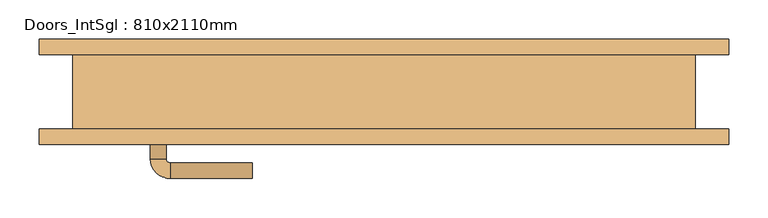
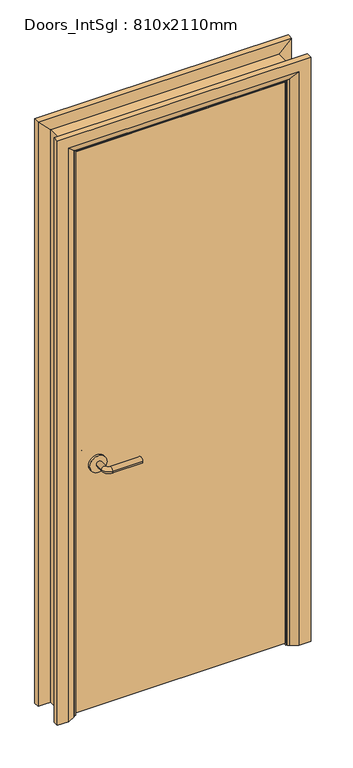
"""IFC4 building model written with IfcOpenShell, lengths in millimetres: door geometry, Doors_IntSgl : 810x2110mm."""

from ifc_helpers import new_model, si_unit, point, frame, frame_2d, origin, place, context, project, spatial, polyline, circle_curve, ellipse_curve, trimmed, segment, composite_curve, outline, extrude, faceted_brep, source, transform, mapped, element, save
from ifc_brep_helpers import plane_surface, cylinder_surface, revolved_surface, advanced_brep


def doors_intsgl_810x2110mm_4fdc4f61(model_context):
    return source(origin(), model_context, "Body", "SolidModel", [
        advanced_brep(
        [(-298.0, -1.5, 900.0), (-278.0, -1.5, 900.0), (-298.0, 28.5, 900.0), (-278.0, 28.5, 900.0), (-273.0, 33.5, 900.0), (-273.0, 53.5, 900.0), (-168.0, 53.5, 900.0), (-168.0, 33.5, 900.0)],
        [
            (0, 1, circle_curve(frame((-288.0, -1.5, 900.0), z_axis=(0.0, -1.0, 0.0), x_axis=(1.0, 0.0, 0.0)), 10.0)),
            (1, 0, circle_curve(frame((-288.0, -1.5, 900.0), z_axis=(0.0, -1.0, 0.0), x_axis=(1.0, 0.0, 0.0)), 10.0)),
            (0, 2),
            (2, 3, circle_curve(frame((-288.0, 28.5, 900.0), z_axis=(0.0, -1.0, 0.0), x_axis=(1.0, 0.0, 0.0)), 10.0)),
            (3, 1),
            (3, 2, circle_curve(frame((-288.0, 28.5, 900.0), z_axis=(0.0, -1.0, 0.0), x_axis=(1.0, 0.0, 0.0)), 10.0)),
            (4, 3, circle_curve(frame((-273.0, 28.5, 900.0), z_axis=(0.0, 0.0, 1.0), x_axis=(-1.0, 0.0, 0.0)), 5.0)),
            (2, 5, circle_curve(frame((-273.0, 28.5, 900.0), z_axis=(0.0, 0.0, -1.0), x_axis=(-1.0, 0.0, 0.0)), 25.0)),
            (5, 4, circle_curve(frame((-273.0, 43.5, 900.0), z_axis=(-1.0, 0.0, 0.0), x_axis=(0.0, -1.0, 0.0)), 10.0)),
            (4, 5, circle_curve(frame((-273.0, 43.5, 900.0), z_axis=(-1.0, 0.0, 0.0), x_axis=(0.0, -1.0, 0.0)), 10.0)),
            (6, 7, circle_curve(frame((-168.0, 43.5, 900.0), z_axis=(1.0, 0.0, 0.0), x_axis=(0.0, -1.0, 0.0)), 10.0)),
            (7, 6, circle_curve(frame((-168.0, 43.5, 900.0), z_axis=(1.0, 0.0, 0.0), x_axis=(0.0, -1.0, 0.0)), 10.0)),
            (5, 6),
            (7, 4),
        ],
        [
            plane_surface(frame((-288.0, -1.5, 900.0), z_axis=(0.0, -1.0, 0.0), x_axis=(0.0, 0.0, 1.0))),
            cylinder_surface(frame((-288.0, -1.5, 900.0), z_axis=(0.0, -1.0, 0.0), x_axis=(1.0, 0.0, 0.0)), 10.0),
            revolved_surface(trimmed(ellipse_curve(frame((-288.0, 28.5, 900.0), z_axis=(0.0, -1.0, 0.0), x_axis=(1.0, 0.0, 0.0)), 10.0, 10.0), [point((-298.0, 28.5, 900.0))], [point((-278.0, 28.5, 900.0))], True, "CARTESIAN"), (-273.0, 28.5, 900.0), (0.0, 0.0, -1.0)),
            revolved_surface(trimmed(ellipse_curve(frame((-288.0, 28.5, 900.0), z_axis=(0.0, -1.0, 0.0), x_axis=(1.0, 0.0, 0.0)), 10.0, 10.0), [point((-278.0, 28.5, 900.0))], [point((-298.0, 28.5, 900.0))], True, "CARTESIAN"), (-273.0, 28.5, 900.0), (0.0, 0.0, -1.0)),
            plane_surface(frame((-168.0, 43.5, 900.0), z_axis=(1.0, 0.0, 0.0), x_axis=(0.0, 0.0, 1.0))),
            cylinder_surface(frame((-273.0, 43.5, 900.0), z_axis=(-1.0, 0.0, 0.0), x_axis=(0.0, -1.0, 0.0)), 10.0),
        ],
        [
            (0, [[1, 2]]),
            (1, [[-1, 3, 4, 5]]),
            (1, [[-2, -5, 6, -3]]),
            (2, [[7, -4, 8, 9]]),
            (3, [[-8, -6, -7, 10]]),
            (4, [[11, 12]]),
            (5, [[-9, 13, -12, 14]]),
            (5, [[-10, -14, -11, -13]]),
        ],
    ),
        extrude(outline(composite_curve([segment(trimmed(circle_curve(frame_2d((900.0, -290.5)), 30.0), [point((900.0, -320.5))], [point((900.0, -260.5))], False, "CARTESIAN"), True, "CONTINUOUS"), segment(trimmed(circle_curve(frame_2d((900.0, -290.5)), 30.0), [point((900.0, -260.5))], [point((900.0, -320.5))], False, "CARTESIAN"), True, "CONTINUOUS")], self_intersect=False)), frame((0.0, -9.5, 0.0), z_axis=(0.0, 1.0, 0.0), x_axis=(0.0, 0.0, 1.0)), (0.0, 0.0, 1.0), 8.0),
        advanced_brep(
        [(-298.0, -55.5, 900.0), (-278.0, -55.5, 900.0), (-278.0, -85.5, 900.0), (-298.0, -85.5, 900.0), (-273.0, -90.5, 900.0), (-273.0, -110.5, 900.0), (-168.0, -110.5, 900.0), (-168.0, -90.5, 900.0)],
        [
            (0, 1, circle_curve(frame((-288.0, -55.5, 900.0), z_axis=(0.0, 1.0, 0.0), x_axis=(1.0, 0.0, 0.0)), 10.0)),
            (1, 0, circle_curve(frame((-288.0, -55.5, 900.0), z_axis=(0.0, 1.0, 0.0), x_axis=(1.0, 0.0, 0.0)), 10.0)),
            (1, 2),
            (2, 3, circle_curve(frame((-288.0, -85.5, 900.0), z_axis=(0.0, 1.0, 0.0), x_axis=(1.0, 0.0, 0.0)), 10.0)),
            (3, 0),
            (3, 2, circle_curve(frame((-288.0, -85.5, 900.0), z_axis=(0.0, 1.0, 0.0), x_axis=(1.0, 0.0, 0.0)), 10.0)),
            (4, 5, circle_curve(frame((-273.0, -100.5, 900.0), z_axis=(-1.0, 0.0, 0.0), x_axis=(0.0, 1.0, 0.0)), 10.0)),
            (5, 3, circle_curve(frame((-273.0, -85.5, 900.0), z_axis=(0.0, 0.0, -1.0), x_axis=(-1.0, 0.0, 0.0)), 25.0)),
            (2, 4, circle_curve(frame((-273.0, -85.5, 900.0), z_axis=(0.0, 0.0, 1.0), x_axis=(-1.0, 0.0, 0.0)), 5.0)),
            (5, 4, circle_curve(frame((-273.0, -100.5, 900.0), z_axis=(-1.0, 0.0, 0.0), x_axis=(0.0, 1.0, 0.0)), 10.0)),
            (6, 7, circle_curve(frame((-168.0, -100.5, 900.0), z_axis=(1.0, 0.0, 0.0), x_axis=(0.0, 1.0, 0.0)), 10.0)),
            (7, 6, circle_curve(frame((-168.0, -100.5, 900.0), z_axis=(1.0, 0.0, 0.0), x_axis=(0.0, 1.0, 0.0)), 10.0)),
            (4, 7),
            (6, 5),
        ],
        [
            plane_surface(frame((-288.0, -55.5, 900.0), z_axis=(0.0, 1.0, 0.0), x_axis=(0.0, 0.0, 1.0))),
            cylinder_surface(frame((-288.0, -55.5, 900.0), z_axis=(0.0, 1.0, 0.0), x_axis=(1.0, 0.0, 0.0)), 10.0),
            revolved_surface(trimmed(ellipse_curve(frame((-288.0, -85.5, 900.0), z_axis=(0.0, -1.0, 0.0), x_axis=(1.0, 0.0, 0.0)), 10.0, 10.0), [point((-298.0, -85.5, 900.0))], [point((-278.0, -85.5, 900.0))], True, "CARTESIAN"), (-273.0, -85.5, 900.0), (0.0, 0.0, -1.0)),
            revolved_surface(trimmed(ellipse_curve(frame((-288.0, -85.5, 900.0), z_axis=(0.0, -1.0, 0.0), x_axis=(1.0, 0.0, 0.0)), 10.0, 10.0), [point((-278.0, -85.5, 900.0))], [point((-298.0, -85.5, 900.0))], True, "CARTESIAN"), (-273.0, -85.5, 900.0), (0.0, 0.0, -1.0)),
            plane_surface(frame((-168.0, -100.5, 900.0), z_axis=(1.0, 0.0, 0.0), x_axis=(0.0, 0.0, 1.0))),
            cylinder_surface(frame((-273.0, -100.5, 900.0), z_axis=(-1.0, 0.0, 0.0), x_axis=(0.0, 1.0, 0.0)), 10.0),
        ],
        [
            (0, [[1, 2]]),
            (1, [[3, 4, 5, -2]]),
            (1, [[-5, 6, -3, -1]]),
            (2, [[7, 8, -4, 9]]),
            (3, [[10, -9, -6, -8]]),
            (4, [[11, 12]]),
            (5, [[13, -11, 14, -7]]),
            (5, [[-14, -12, -13, -10]]),
        ],
    ),
        extrude(outline(composite_curve([segment(trimmed(circle_curve(frame_2d((900.0, -290.5)), 30.0), [point((900.0, -320.5))], [point((900.0, -260.5))], False, "CARTESIAN"), True, "CONTINUOUS"), segment(trimmed(circle_curve(frame_2d((900.0, -290.5)), 30.0), [point((900.0, -260.5))], [point((900.0, -320.5))], False, "CARTESIAN"), True, "CONTINUOUS")], self_intersect=False)), frame((0.0, -55.5, 0.0), z_axis=(0.0, 1.0, 0.0), x_axis=(0.0, 0.0, 1.0)), (0.0, 0.0, 1.0), 8.0),
        extrude(outline(polyline([(363.0, -9.5), (363.0, -47.5), (-363.0, -47.5), (-363.0, -9.5), (363.0, -9.5)])), frame((0.0, 0.0, 8.0), z_axis=(0.0, 0.0, 1.0), x_axis=(1.0, 0.0, 0.0)), (0.0, 0.0, 1.0), 2060.0),
        advanced_brep(
        [(440.0, -67.5, 0.0), (400.0, -67.5, 0.0), (374.0, -53.5, 0.0), (370.0, -47.5, 0.0), (440.0, -47.5, 0.0), (440.0, -47.5, 2145.0), (440.0, -67.5, 2145.0), (370.0, -47.5, 2075.0), (-370.0, -47.5, 2075.0), (-370.0, -47.5, 0.0), (-440.0, -47.5, 0.0), (-440.0, -47.5, 2145.0), (374.0, -53.5, 2079.0), (400.0, -67.5, 2105.0), (-440.0, -67.5, 2145.0), (-440.0, -67.5, 0.0), (-400.0, -67.5, 0.0), (-400.0, -67.5, 2105.0), (-374.0, -53.5, 2079.0), (-374.0, -53.5, 0.0)],
        [
            (0, 1),
            (1, 2),
            (2, 3, circle_curve(frame((378.0, -46.5, 0.0), z_axis=(0.0, 0.0, -1.0), x_axis=(1.0, 0.0, 0.0)), 8.0622577)),
            (3, 4),
            (4, 0),
            (4, 5),
            (5, 6),
            (6, 0),
            (3, 7),
            (7, 8),
            (8, 9),
            (9, 10),
            (10, 11),
            (11, 5),
            (2, 12),
            (12, 7, ellipse_curve(frame((378.0, -46.5, 2083.0), z_axis=(0.7071067811865475, 0.0, -0.7071067811865475), x_axis=(-0.7071067811865474, 0.0, -0.7071067811865476)), 11.4017543, 8.0622577)),
            (1, 13),
            (13, 12),
            (6, 14),
            (14, 15),
            (15, 16),
            (16, 17),
            (17, 13),
            (11, 14),
            (12, 18),
            (18, 8, ellipse_curve(frame((-378.0, -46.5, 2083.0), z_axis=(0.7071067811865475, 0.0, 0.7071067811865475), x_axis=(0.7071067811865476, 0.0, -0.7071067811865474)), 11.4017543, 8.0622577)),
            (17, 18),
            (15, 10),
            (9, 19, circle_curve(frame((-378.0, -46.5, 0.0), z_axis=(0.0, 0.0, -1.0), x_axis=(-1.0, 0.0, 0.0)), 8.0622577)),
            (19, 16),
            (18, 19),
        ],
        [
            plane_surface(frame((370.0, -47.5, 0.0), z_axis=(0.0, 0.0, -1.0), x_axis=(0.0, 1.0, 0.0))),
            plane_surface(frame((440.0, -67.5, 0.0), z_axis=(1.0, 0.0, 0.0), x_axis=(0.0, 0.0, 1.0))),
            plane_surface(frame((440.0, -47.5, 0.0), z_axis=(0.0, 1.0, 0.0), x_axis=(0.0, 0.0, 1.0))),
            cylinder_surface(frame((378.0, -46.5, 0.0), z_axis=(0.0, 0.0, -1.0), x_axis=(1.0, 0.0, 0.0)), 8.0622577),
            plane_surface(frame((374.0, -53.5, 0.0), z_axis=(-0.4740998230350126, -0.880471099922178, 0.0), x_axis=(0.0, 0.0, 1.0))),
            plane_surface(frame((400.0, -67.5, 0.0), z_axis=(0.0, -1.0, 0.0), x_axis=(0.0, 0.0, 1.0))),
            plane_surface(frame((440.0, -67.5, 2145.0), z_axis=(0.0, 0.0, 1.0), x_axis=(-1.0, 0.0, 0.0))),
            cylinder_surface(frame((370.0, -46.5, 2083.0), z_axis=(1.0, 0.0, 0.0), x_axis=(0.0, 0.0, 1.0)), 8.0622577),
            plane_surface(frame((374.0, -53.5, 2079.0), z_axis=(0.0, -0.8804710999221764, -0.4740998230350154), x_axis=(-1.0, 0.0, 0.0))),
            plane_surface(frame((-370.0, -47.5, 0.0), z_axis=(0.0, 0.0, -1.0), x_axis=(0.0, 1.0, 0.0))),
            plane_surface(frame((-440.0, -67.5, 2145.0), z_axis=(-1.0, 0.0, 0.0), x_axis=(0.0, 0.0, -1.0))),
            cylinder_surface(frame((-378.0, -46.5, 2075.0), z_axis=(0.0, 0.0, 1.0), x_axis=(-1.0, 0.0, 0.0)), 8.0622577),
            plane_surface(frame((-374.0, -53.5, 2079.0), z_axis=(0.47409982303501824, -0.8804710999221749, 0.0), x_axis=(0.0, 0.0, -1.0))),
        ],
        [
            (0, [[1, 2, 3, 4, 5]]),
            (1, [[6, 7, 8, -5]]),
            (2, [[9, 10, 11, 12, 13, 14, -6, -4]]),
            (3, [[15, 16, -9, -3]]),
            (4, [[17, 18, -15, -2]]),
            (5, [[-8, 19, 20, 21, 22, 23, -17, -1]]),
            (6, [[-14, 24, -19, -7]]),
            (7, [[25, 26, -10, -16]]),
            (8, [[-23, 27, -25, -18]]),
            (9, [[28, -12, 29, 30, -21]]),
            (10, [[-13, -28, -20, -24]]),
            (11, [[31, -29, -11, -26]]),
            (12, [[-22, -30, -31, -27]]),
        ],
    ),
        extrude(outline(polyline([(0.0, -346.0), (2051.0, -346.0), (2051.0, 346.0), (0.0, 346.0), (0.0, 365.0), (2070.0, 365.0), (2070.0, -365.0), (0.0, -365.0), (0.0, -346.0)])), frame((0.0, -7.5, 0.0), z_axis=(0.0, 1.0, 0.0), x_axis=(0.0, 0.0, 1.0)), (0.0, 0.0, 1.0), 32.0),
        advanced_brep(
        [(-440.0, 67.5, 0.0), (-400.0, 67.5, 0.0), (-374.0, 53.5, 0.0), (-370.0, 47.5, 0.0), (-440.0, 47.5, 0.0), (-440.0, 47.5, 2145.0), (-440.0, 67.5, 2145.0), (-370.0, 47.5, 2075.0), (-374.0, 53.5, 2079.0), (-400.0, 67.5, 2105.0), (440.0, 47.5, 2145.0), (440.0, 67.5, 2145.0), (370.0, 47.5, 2075.0), (374.0, 53.5, 2079.0), (400.0, 67.5, 2105.0), (440.0, 67.5, 0.0), (440.0, 47.5, 0.0), (370.0, 47.5, 0.0), (374.0, 53.5, 0.0), (400.0, 67.5, 0.0)],
        [
            (0, 1),
            (1, 2),
            (2, 3, circle_curve(frame((-378.0, 46.5, 0.0), z_axis=(0.0, 0.0, -1.0), x_axis=(-1.0, 0.0, 0.0)), 8.0622577)),
            (3, 4),
            (4, 0),
            (4, 5),
            (5, 6),
            (6, 0),
            (3, 7),
            (7, 5),
            (2, 8),
            (8, 7, ellipse_curve(frame((-378.0, 46.5, 2083.0), z_axis=(-0.7071067811865475, 0.0, -0.7071067811865475), x_axis=(0.7071067811865474, 0.0, -0.7071067811865476)), 11.4017543, 8.0622577)),
            (1, 9),
            (9, 8),
            (6, 9),
            (5, 10),
            (10, 11),
            (11, 6),
            (7, 12),
            (12, 10),
            (8, 13),
            (13, 12, ellipse_curve(frame((378.0, 46.5, 2083.0), z_axis=(-0.7071067811865475, 0.0, 0.7071067811865475), x_axis=(-0.7071067811865476, 0.0, -0.7071067811865474)), 11.4017543, 8.0622577)),
            (9, 14),
            (14, 13),
            (11, 14),
            (15, 16),
            (16, 17),
            (17, 18, circle_curve(frame((378.0, 46.5, 0.0), z_axis=(0.0, 0.0, -1.0), x_axis=(1.0, 0.0, 0.0)), 8.0622577)),
            (18, 19),
            (19, 15),
            (10, 16),
            (15, 11),
            (12, 17),
            (13, 18),
            (14, 19),
        ],
        [
            plane_surface(frame((-370.0, 120.3010989, 0.0), z_axis=(0.0, 0.0, -1.0), x_axis=(1.0, 0.0, 0.0))),
            plane_surface(frame((-440.0, 67.5, 0.0), z_axis=(-1.0, 0.0, 0.0), x_axis=(0.0, 0.0, 1.0))),
            plane_surface(frame((-440.0, 47.5, 0.0), z_axis=(0.0, -1.0, 0.0), x_axis=(0.0, 0.0, 1.0))),
            cylinder_surface(frame((-378.0, 46.5, 0.0), z_axis=(0.0, 0.0, -1.0), x_axis=(-1.0, 0.0, 0.0)), 8.0622577),
            plane_surface(frame((-374.0, 53.5, 0.0), z_axis=(0.4740998230350183, 0.8804710999221749, 0.0), x_axis=(0.0, 0.0, 1.0))),
            plane_surface(frame((-400.0, 67.5, 0.0), z_axis=(0.0, 1.0, 0.0), x_axis=(0.0, 0.0, 1.0))),
            plane_surface(frame((-440.0, 67.5, 2145.0), z_axis=(0.0, 0.0, 1.0), x_axis=(1.0, 0.0, 0.0))),
            plane_surface(frame((-440.0, 47.5, 2145.0), z_axis=(0.0, -1.0, 0.0), x_axis=(1.0, 0.0, 0.0))),
            cylinder_surface(frame((-370.0, 46.5, 2083.0), z_axis=(-1.0, 0.0, 0.0), x_axis=(0.0, 0.0, 1.0)), 8.0622577),
            plane_surface(frame((-374.0, 53.5, 2079.0), z_axis=(0.0, 0.8804710999221749, -0.4740998230350183), x_axis=(1.0, 0.0, 0.0))),
            plane_surface(frame((-400.0, 67.5, 2105.0), z_axis=(0.0, 1.0, 0.0), x_axis=(1.0, 0.0, 0.0))),
            plane_surface(frame((370.0, 120.3010989, 0.0), z_axis=(0.0, 0.0, -1.0), x_axis=(-1.0, 0.0, 0.0))),
            plane_surface(frame((440.0, 67.5, 2145.0), z_axis=(1.0, 0.0, 0.0), x_axis=(0.0, 0.0, -1.0))),
            plane_surface(frame((440.0, 47.5, 2145.0), z_axis=(0.0, -1.0, 0.0), x_axis=(0.0, 0.0, -1.0))),
            cylinder_surface(frame((378.0, 46.5, 2075.0), z_axis=(0.0, 0.0, 1.0), x_axis=(1.0, 0.0, 0.0)), 8.0622577),
            plane_surface(frame((374.0, 53.5, 2079.0), z_axis=(-0.4740998230350183, 0.8804710999221749, 0.0), x_axis=(0.0, 0.0, -1.0))),
            plane_surface(frame((400.0, 67.5, 2105.0), z_axis=(0.0, 1.0, 0.0), x_axis=(0.0, 0.0, -1.0))),
        ],
        [
            (0, [[1, 2, 3, 4, 5]]),
            (1, [[6, 7, 8, -5]]),
            (2, [[9, 10, -6, -4]]),
            (3, [[11, 12, -9, -3]]),
            (4, [[13, 14, -11, -2]]),
            (5, [[-8, 15, -13, -1]]),
            (6, [[16, 17, 18, -7]]),
            (7, [[19, 20, -16, -10]]),
            (8, [[21, 22, -19, -12]]),
            (9, [[23, 24, -21, -14]]),
            (10, [[-18, 25, -23, -15]]),
            (11, [[26, 27, 28, 29, 30]]),
            (12, [[31, -26, 32, -17]]),
            (13, [[33, -27, -31, -20]]),
            (14, [[34, -28, -33, -22]]),
            (15, [[35, -29, -34, -24]]),
            (16, [[-32, -30, -35, -25]]),
        ],
    ),
        faceted_brep([(-365.0, -47.5, 0.0), (-397.0, -47.5, 0.0), (-397.0, 47.5, 0.0), (-365.0, 47.5, 0.0), (-365.0, 47.5, 2070.0), (-365.0, -47.5, 2070.0), (-397.0, 47.5, 2102.0), (-397.0, -47.5, 2102.0), (365.0, 47.5, 2070.0), (365.0, -47.5, 2070.0), (397.0, 47.5, 2102.0), (397.0, -47.5, 2102.0), (365.0, -47.5, 0.0), (365.0, 47.5, 0.0), (397.0, 47.5, 0.0), (397.0, -47.5, 0.0)], [[[0, 1, 2, 3]], [[3, 4, 5, 0]], [[2, 6, 4, 3]], [[1, 7, 6, 2]], [[0, 5, 7, 1]], [[4, 8, 9, 5]], [[6, 10, 8, 4]], [[7, 11, 10, 6]], [[5, 9, 11, 7]], [[12, 13, 14, 15]], [[8, 13, 12, 9]], [[10, 14, 13, 8]], [[11, 15, 14, 10]], [[9, 12, 15, 11]]]),
    ])


if __name__ == "__main__":
    model = new_model("IFC4")
    model_context = context("Model", 3, world=origin())
    ifc_project = project(units=[si_unit("LENGTHUNIT", "METRE", prefix="MILLI")], contexts=[model_context])
    site = spatial("IfcSite", under=ifc_project)
    building = spatial("IfcBuilding", under=site)
    placement = place(None, origin())
    doors_intsgl_810x2110mm_shape = doors_intsgl_810x2110mm_4fdc4f61(model_context)
    element("IfcDoor", 1, ObjectType="Doors_IntSgl : 810x2110mm", at=placement, inside=building, context=model_context, shape_type="MappedRepresentation", body=[
        mapped(doors_intsgl_810x2110mm_shape, transform((0.0, 0.0, 0.0), x_axis=(1.0, 0.0, 0.0), y_axis=(0.0, 1.0, 0.0), z_axis=(0.0, 0.0, 1.0))),
    ])
    save(model, "model.ifc")

# Revit data of these elements
# Type "Doors_IntSgl : 810x2110mm"
#   Construction Type Id = "MDOOR"
#   Type Mark = "42"
#   Type Comments = "Internal Single"
#   Operation = "SingleSwingRight"
#   Manufacturer = "Revit"
#   Keynote = "L20"
#   Description = "Internal Single Door"
#   Analytic Construction = "Metal"
#   UnderCut = 8 mm
#   Tolerance = 2 mm
#   Thickness = 38 mm
#   Thermal Resistance (R) = 0.270117 (m²·K)/W
#   Structural Tolerance = 8 mm
#   StopDepth = 32 mm
#   Stop Thickness = 19 mm
#   Rough Width = 810 mm
#   Rough Height = 2110 mm
#   Height to Top Lock Rail = 1000 mm
#   Heat Transfer Coefficient (U) = 3.7021 W/(m²·K)
#   Handle Z Distance = 900 mm
#   Handle X Distance = 75 mm
#   Frame Thickness = 32 mm
#   Door Panel Width = 726 mm
#   Door Panel Thickness = 38 mm
#   Door Panel Offset = 0 mm
#   Height = 2110 mm
#   Width = 810 mm
#   Door Panel Height = 2060 mm
#   Architrave Setback = 5 mm
#   Vis - Ironmongery = yes
#   Material Ironmongery = Door - Handle
#   Material Frame = Door - Frame/Mullion (1)
#   Material Door = Door - Panel
#   Material Architrave = Door - Architrave
#   Visual Light Transmittance = 0
#   Solar Heat Gain Coefficient = 0
#   Function = (empty or 0)
#   Wall Closure = (empty or 0)
# Element 1 (IfcDoor, "Doors_IntSgl : 810x2110mm")
#   Materials on its faces: "Door - Architrave", "Door - Handle", "Door - Frame/Mullion (1)", "Door - Panel"
# Materials
#   "Door - Handle": class "Miscellaneous", colour RGB 0 0 0, transparency 0, Keynote = "P21"
#   "Door - Frame/Mullion (1)": class "Wood", colour RGB 212 179 113, transparency 0, Keynote = "L20", Cost = 0
#   "Door - Panel": class "Wood", colour RGB 210 159 95, transparency 0, Keynote = "L20"
#   "Door - Architrave": class "Wood", colour RGB 154 90 5, transparency 0, Keynote = "P20"
